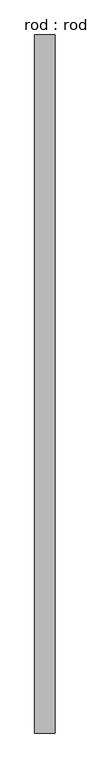
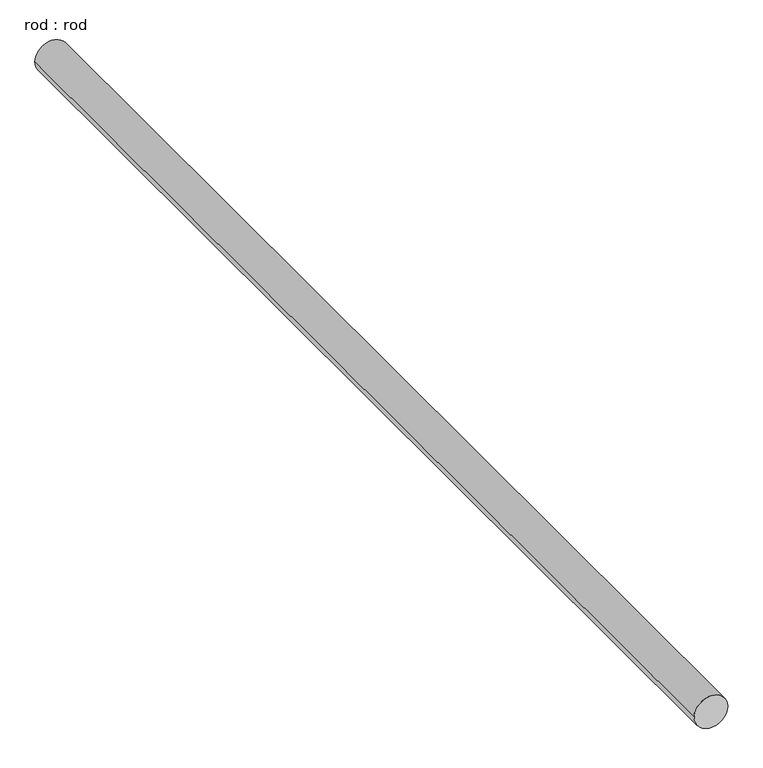
"""IFC4 building model written with IfcOpenShell, lengths in millimetres: proxy geometry, rod : rod."""

from ifc_helpers import new_model, si_unit, point, frame, frame_2d, origin, place, context, project, spatial, circle_curve, trimmed, segment, composite_curve, outline, extrude, source, transform, mapped, element, save


def rod_rod_8bb489ba(model_context):
    return source(origin(), model_context, "Body", "SweptSolid", [
        extrude(outline(composite_curve([segment(trimmed(circle_curve(frame_2d((0.0108462, 0.0)), 200.0), [point((0.0108462, 200.0))], [point((0.0108462, -200.0))], False, "CARTESIAN"), True, "CONTINUOUS"), segment(trimmed(circle_curve(frame_2d((0.0108462, 0.0)), 200.0), [point((0.0108462, -200.0))], [point((0.0108462, 200.0))], False, "CARTESIAN"), True, "CONTINUOUS")], self_intersect=False)), frame((0.0, -2724.2356704, 0.0), z_axis=(0.0, 1.0, 0.0), x_axis=(0.0, 0.0, 1.0)), (0.0, 0.0, 1.0), 13633.9285714),
    ])


if __name__ == "__main__":
    model = new_model("IFC4")
    model_context = context("Model", 3, world=origin())
    ifc_project = project(units=[si_unit("LENGTHUNIT", "METRE", prefix="MILLI")], contexts=[model_context])
    site = spatial("IfcSite", under=ifc_project)
    building = spatial("IfcBuilding", under=site)
    placement = place(None, origin())
    rod_rod_shape = rod_rod_8bb489ba(model_context)
    element("IfcBuildingElementProxy", 1, Name="rod : rod", ObjectType="rod : rod", at=placement, inside=building, context=model_context, shape_type="MappedRepresentation", body=[
        mapped(rod_rod_shape, transform((0.0, 0.0, 0.0), x_axis=(1.0, 0.0, 0.0), y_axis=(0.0, 1.0, 0.0), z_axis=(0.0, 0.0, 1.0))),
    ])
    save(model, "model.ifc")

# Revit data of these elements
# Type "rod : rod"
#   Default Elevation = 0
